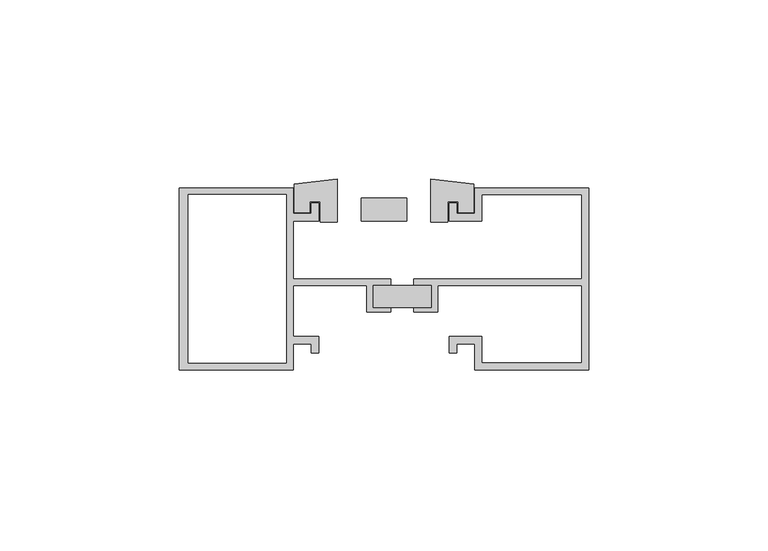
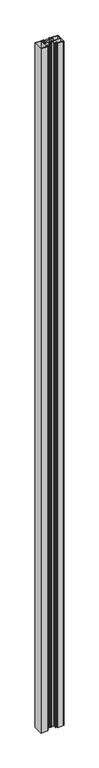
"""IFC4 building model written with IfcOpenShell, lengths in millimetres: proxy geometry, Generic Models 3:Generic Models 1:5:Generic Models 1:5 : Generic Models 3:Generic Models 1:300625:345888:Generic Models 1:5:Generic Models 1:5 : Generic Models 3:Generic Models 1:300625:345888 : Generic Models 3:Generic Models 1:5:Generic Models 1:5 : Generic Models 3:Generic Models 1:300625:345888:1 : Generic Models 3:Generic Models 1:5:Generic Models 1:5 : Generic Models 3:Generic Models 1:300625:345888:Generic Models 1:5:Generic Models 1:5 : Generic Models 3:Generic Models 1:300625:345888 : Generic Models 3:Generic Models 1:5:Generic Models 1:5 : Generic Models 3:Generic Models 1:300625:345888:301574."""

from ifc_helpers import new_model, si_unit, frame, origin, place, context, project, spatial, polyline, outline, extrude, source, transform, mapped, element, save


def generic_models_d13590e7(model_context):
    return source(origin(), model_context, "Body", "SweptSolid", [
        extrude(outline(polyline([(560302.3728277, -573543.2294825), (560318.4842638, -573543.2294825), (560318.4842638, -573549.3092697), (560302.3728277, -573549.3092697), (560302.3728277, -573543.2294825)])), frame((0.0, 0.0, 66.3122056), z_axis=(0.0, 0.0, 1.0), x_axis=(1.0, 0.0, 0.0)), (0.0, 0.0, 1.0), 3584.971571),
        extrude(outline(polyline([(560298.9867239, -573518.7985671), (560311.6867239, -573518.7985671), (560311.6867239, -573525.1421155), (560298.9867239, -573525.1421155), (560298.9867239, -573518.7985671)])), frame((0.0, 0.0, 66.3122056), z_axis=(0.0, 0.0, 1.0), x_axis=(1.0, 0.0, 0.0)), (0.0, 0.0, 1.0), 3584.971571),
        extrude(outline(polyline([(560287.4942372, -573519.8254499), (560284.648559, -573519.8254499), (560284.648559, -573522.7693096), (560280.3504872, -573522.7693096), (560280.3504872, -573514.9296002), (560292.2482931, -573513.4687334), (560292.2482931, -573525.5389905), (560287.4942372, -573525.5389905), (560287.4942372, -573519.8254499)])), frame((0.0, 0.0, 66.3122056), z_axis=(0.0, 0.0, 1.0), x_axis=(1.0, 0.0, 0.0)), (0.0, 0.0, 1.0), 3584.971571),
        extrude(outline(polyline([(560330.3229606, -573514.9296002), (560330.3229606, -573522.7693096), (560326.0248888, -573522.7693096), (560326.0248888, -573519.8254499), (560323.1792106, -573519.8254499), (560323.1792106, -573525.5389905), (560318.4251548, -573525.5389905), (560318.4251548, -573513.4687333), (560330.3229606, -573514.9296002)])), frame((0.0, 0.0, 66.3122056), z_axis=(0.0, 0.0, 1.0), x_axis=(1.0, 0.0, 0.0)), (0.0, 0.0, 1.0), 3584.9377944),
        extrude(outline(polyline([(560248.1867239, -573566.7126607), (560248.1867239, -573515.9464373), (560279.9536122, -573515.9464373), (560279.9536122, -573523.1661846), (560285.045434, -573523.1661846), (560285.045434, -573520.2223249), (560287.0973622, -573520.2223249), (560287.0973622, -573525.1421155), (560279.9536122, -573525.1421155), (560279.9536122, -573541.329549), (560307.2366574, -573541.329549), (560307.2366574, -573543.2294825), (560302.3728277, -573543.2294825), (560302.3728277, -573549.3092697), (560307.2366574, -573549.3092697), (560307.2366574, -573550.6012245), (560300.4728941, -573550.6012245), (560300.4728941, -573543.2294825), (560279.9536122, -573543.2294825), (560279.9536122, -573557.4409852), (560287.0973622, -573557.4409852), (560287.0973622, -573562.0121448), (560285.045434, -573562.0121448), (560285.045434, -573559.4929133), (560279.9536122, -573559.4929133), (560279.9536122, -573566.7126607), (560248.1867239, -573566.7126607)]), holes=[polyline([(560278.0536787, -573517.8463708), (560250.6946362, -573517.8463708), (560250.6946362, -573564.8127272), (560278.0536787, -573564.8127272), (560278.0536787, -573517.8463708)])]), frame((0.0, 0.0, 66.3122056), z_axis=(0.0, 0.0, 1.0), x_axis=(1.0, 0.0, 0.0)), (0.0, 0.0, 1.0), 3584.971571),
        extrude(outline(polyline([(560325.6280138, -573520.2223249), (560325.6280138, -573523.1661846), (560330.7198356, -573523.1661846), (560330.7198356, -573515.9464373), (560362.4867239, -573515.9464373), (560362.4867239, -573566.7126607), (560330.7198356, -573566.7126607), (560330.7198356, -573559.4929133), (560325.6280138, -573559.4929133), (560325.6280138, -573562.0121448), (560323.5760856, -573562.0121448), (560323.5760856, -573557.4409852), (560332.6197691, -573557.4409852), (560332.6197691, -573564.7904481), (560360.5107931, -573564.7904481), (560360.5107931, -573543.2294825), (560320.3841973, -573543.2294825), (560320.3841973, -573550.6012245), (560313.620434, -573550.6012245), (560313.620434, -573549.3092697), (560318.4842638, -573549.3092697), (560318.4842638, -573543.2294825), (560313.620434, -573543.2294825), (560313.620434, -573541.329549), (560360.5107931, -573541.329549), (560360.5107931, -573517.8562363), (560332.6197691, -573517.8562363), (560332.6197691, -573525.1421155), (560323.5760856, -573525.1421155), (560323.5760856, -573520.2223249), (560325.6280138, -573520.2223249)])), frame((0.0, 0.0, 66.3122056), z_axis=(0.0, 0.0, 1.0), x_axis=(1.0, 0.0, 0.0)), (0.0, 0.0, 1.0), 3584.971571),
    ])


if __name__ == "__main__":
    model = new_model("IFC4")
    model_context = context("Model", 3, world=origin())
    ifc_project = project(units=[si_unit("LENGTHUNIT", "METRE", prefix="MILLI")], contexts=[model_context])
    site = spatial("IfcSite", under=ifc_project)
    building = spatial("IfcBuilding", under=site)
    placement = place(None, origin())
    generic_models_shape = generic_models_d13590e7(model_context)
    element("IfcBuildingElementProxy", 1, Name="Generic Models 3:Generic Models 1:5:Generic Models 1:5 : Generic Models 3:Generic Models 1:300625:345888:Generic Models 1:5:Generic Models 1:5 : Generic Models 3:Generic Models 1:300625:345888 : Generic Models 3:Generic Models 1:5:Generic Models 1:5 : Generic Models 3:Generic Models 1:300625:345888:1 : Generic Models 3:Generic Models 1:5:Generic Models 1:5 : Generic Models 3:Generic Models 1:300625:345888:Generic Models 1:5:Generic Models 1:5 : Generic Models 3:Generic Models 1:300625:345888 : Generic Models 3:Generic Models 1:5:Generic Models 1:5 : Generic Models 3:Generic Models 1:300625:345888:301574", ObjectType="Generic Models 3:Generic Models 1:5:Generic Models 1:5 : Generic Models 3:Generic Models 1:300625:345888:Generic Models 1:5:Generic Models 1:5 : Generic Models 3:Generic Models 1:300625:345888 : Generic Models 3:Generic Models 1:5:Generic Models 1:5 : Generic Models 3:Generic Models 1:300625:345888:1 : Generic Models 3:Generic Models 1:5:Generic Models 1:5 : Generic Models 3:Generic Models 1:300625:345888:Generic Models 1:5:Generic Models 1:5 : Generic Models 3:Generic Models 1:300625:345888 : Generic Models 3:Generic Models 1:5:Generic Models 1:5 : Generic Models 3:Generic Models 1:300625:345888:301574", at=placement, inside=building, context=model_context, shape_type="MappedRepresentation", body=[
        mapped(generic_models_shape, transform((0.0, 0.0, 0.0), x_axis=(1.0, 0.0, 0.0), y_axis=(0.0, 1.0, 0.0), z_axis=(0.0, 0.0, 1.0))),
    ])
    save(model, "model.ifc")

# Revit data of these elements
# Type "Generic Models 3:Generic Models 1:5:Generic Models 1:5 : Generic Models 3:Generic Models 1:300625:345888:Generic Models 1:5:Generic Models 1:5 : Generic Models 3:Generic Models 1:300625:345888 : Generic Models 3:Generic Models 1:5:Generic Models 1:5 : Generic Models 3:Generic Models 1:300625:345888:1 : Generic Models 3:Generic Models 1:5:Generic Models 1:5 : Generic Models 3:Generic Models 1:300625:345888:Generic Models 1:5:Generic Models 1:5 : Generic Models 3:Generic Models 1:300625:345888 : Generic Models 3:Generic Models 1:5:Generic Models 1:5 : Generic Models 3:Generic Models 1:300625:345888:301574"
#   NameOverride = "Generic Models 3:Generic Models 1:5:Generic Models 1:5 : Generic Models 3:Generic Models 1:300625:345888:Generic Models 1:5:Generic Models 1:5 : Generic Models 3:Generic Models 1:300625:345888 : Generic Models 3:Generic Models 1:5:Generic Models 1:5 : Generic Models 3:Generic Models 1:300625:345888:301574"
#   ObjectTypeOverride = "Generic Models 1:5:Generic Models 1:5 : Generic Models 3:Generic Models 1:300625:345888 : Generic Models 3:Generic Models 1:5:Generic Models 1:5 : Generic Models 3:Generic Models 1:300625:345888"
#   Reference = "Generic Models 1"
#   Tag = "301574"
# Element 1 (IfcBuildingElementProxy, "Generic Models 3:Generic Models 1:5:Generic Models 1:5 : Generic Models 3:Generic Models 1:300625:345888:Generic Models 1:5:Generic Models 1:5 : Generic Models 3:Generic Models 1:300625:345888 : Generic Models 3:Generic Models 1:5:Generic Models 1:5 : Generic Models 3:Generic Models 1:300625:345888:1 : Generic Models 3:Generic Models 1:5:Generic Models 1:5 : Generic Models 3:Generic Models 1:300625:345888:Generic Models 1:5:Generic Models 1:5 : Generic Models 3:Generic Models 1:300625:345888 : Generic Models 3:Generic Models 1:5:Generic Models 1:5 : Generic Models 3:Generic Models 1:300625:345888:301574")
#   Materials on its faces: "THERMAL BROKEN ALUMINUM STOREFRONT"
# Materials
#   "THERMAL BROKEN ALUMINUM STOREFRONT": class "Unassigned", colour RGB 244 244 244, transparency 0, Cost = 0
